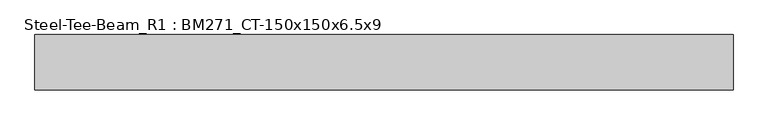
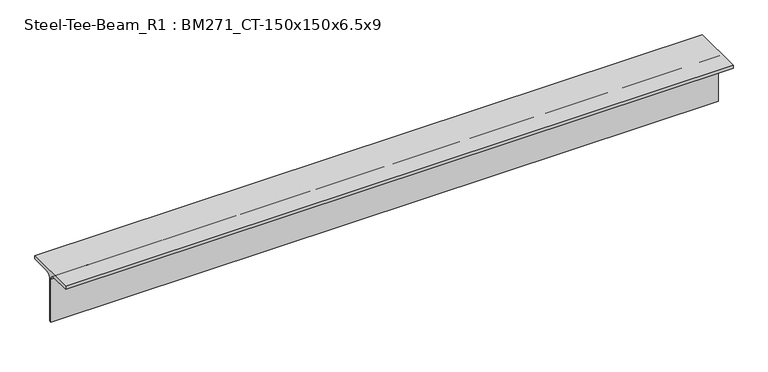
"""IFC4 building model written with IfcOpenShell, lengths in millimetres: member geometry, Steel-Tee-Beam_R1 : BM271_CT-150x150x6.5x9."""

from ifc_helpers import new_model, si_unit, point, frame, frame_2d, origin, place, context, project, spatial, polyline, circle_curve, trimmed, segment, composite_curve, outline, extrude, source, transform, mapped, element, save


def steel_tee_beam_r1_bm271_ct_150x150x6_5x9_964af9dc(model_context):
    return source(origin(), model_context, "Body", "SweptSolid", [
        extrude(outline(composite_curve([segment(polyline([(-75.0, 75.0), (75.0, 75.0), (75.0, 66.0), (16.25, 66.0)]), True, "CONTINUOUS"), segment(trimmed(circle_curve(frame_2d((16.25, 53.0)), 13.0), [point((16.25, 66.0))], [point((3.25, 53.0))], True, "CARTESIAN"), True, "CONTINUOUS"), segment(polyline([(3.25, 53.0), (3.25, -75.0), (-3.25, -75.0), (-3.25, 53.0)]), True, "CONTINUOUS"), segment(trimmed(circle_curve(frame_2d((-16.25, 53.0)), 13.0), [point((-3.25, 53.0))], [point((-16.25, 66.0))], True, "CARTESIAN"), True, "CONTINUOUS"), segment(polyline([(-16.25, 66.0), (-75.0, 66.0), (-75.0, 75.0)]), True, "CONTINUOUS")], self_intersect=False)), frame((-983.9814396, 0.0, 0.0), z_axis=(1.0, 0.0, 0.0), x_axis=(0.0, 1.0, 0.0)), (0.0, 0.0, 1.0), 1884.11033),
    ])


if __name__ == "__main__":
    model = new_model("IFC4")
    model_context = context("Model", 3, world=origin())
    ifc_project = project(units=[si_unit("LENGTHUNIT", "METRE", prefix="MILLI")], contexts=[model_context])
    site = spatial("IfcSite", under=ifc_project)
    building = spatial("IfcBuilding", under=site)
    placement = place(None, origin())
    steel_tee_beam_r1_bm271_ct_150x150x6_5x9_shape = steel_tee_beam_r1_bm271_ct_150x150x6_5x9_964af9dc(model_context)
    element("IfcMember", 1, ObjectType="Steel-Tee-Beam_R1 : BM271_CT-150x150x6.5x9", at=placement, inside=building, context=model_context, shape_type="MappedRepresentation", body=[
        mapped(steel_tee_beam_r1_bm271_ct_150x150x6_5x9_shape, transform((0.0, 0.0, 0.0), x_axis=(1.0, 0.0, 0.0), y_axis=(0.0, 1.0, 0.0), z_axis=(0.0, 0.0, 1.0))),
    ])
    save(model, "model.ifc")

# Revit data of these elements
# Type "Steel-Tee-Beam_R1 : BM271_CT-150x150x6.5x9"
#   Keynote = "CT-150x150x6.5x9"
#   Surface Area = 0.588841 m²/m
#   Section Area = 23.3904 cm²
#   Mass per Unit Length = 18.3614 kg/m
#   Length [instance default] = 1.5240 m
#   bf = 0.1500 m
#   d = 0.1500 m
#   k = 0.0220 m
#   r = 0.0130 m
#   tf = 0.0090 m
#   tw = 0.0065 m
#   hec_material4 [instance default] = none
#   hec_material3 [instance default] = none
#   hec_material2 [instance default] = none
#   hec_material1 [instance default] = none
#   Structural Material [instance default] = Steel, 45-345
#   Assembly Code = ""
# Element 1 (IfcMember, "Steel-Tee-Beam_R1 : BM271_CT-150x150x6.5x9")
#   Structural Material = none
# Materials
#   "Steel, 45-345": class "Metal", colour RGB 189 187 185, transparency 0, Description = "Steel 345 MPa", Cost = 0
